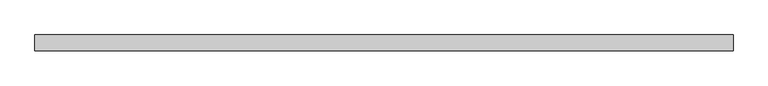
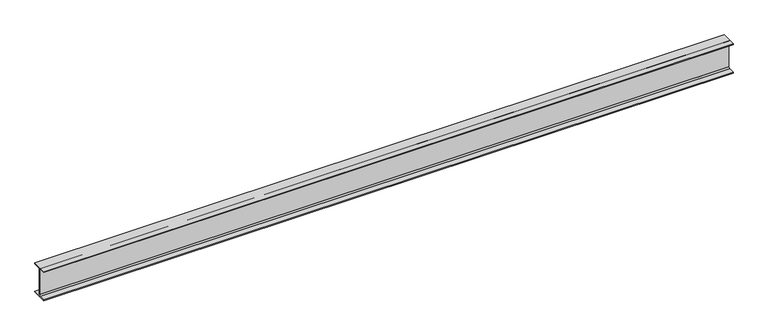
"""IFC4 building model written with IfcOpenShell, lengths in millimetres: beam geometry, Steel Framing_H_KS : H_SB_AR_S02_H-300x150x6.5x9_SRG3."""

import ifcopenshell
import ifcopenshell.guid

model = None  # the IFC model being written
_history = None  # IfcOwnerHistory: only IFC2X3 demands one
_inside = {}  # id of a spatial element -> (the spatial element, [elements in it])
_under = {}  # id of a project, library or spatial element -> (it, [spatial elements below it])
_declared = {}  # id of a project -> (the project, [libraries it declares])
_typed = {}  # id of a type object -> (the type object, [elements of that type])
_made_of = {}  # id of a material, layer set ... -> (it, [elements and type objects made of it])


def new_model(schema):
    """Start an empty IFC model of exactly this schema.

    Asked for "IFC4X3", IfcOpenShell would pick the latest addendum, in which some entities
    have other attributes; the version numbers below select the first issue.
    IFC2X3 requires an IfcOwnerHistory on every rooted entity: one is made here for all.
    """
    global model, _history
    if schema == "IFC4X3":
        model = ifcopenshell.file(schema_version=(4, 3, 0, 0))
    else:
        model = ifcopenshell.file(schema=schema)
    _inside.clear()
    _under.clear()
    _declared.clear()
    _typed.clear()
    _made_of.clear()
    _history = None
    if model.schema == "IFC2X3":
        org = make("IfcOrganization", Name="unknown")
        user = make(
            "IfcPersonAndOrganization",
            ThePerson=make("IfcPerson", FamilyName="unknown"),
            TheOrganization=org,
        )
        app = make(
            "IfcApplication",
            ApplicationDeveloper=org,
            Version="unknown",
            ApplicationFullName="unknown",
            ApplicationIdentifier="unknown",
        )
        _history = make(
            "IfcOwnerHistory",
            OwningUser=user,
            OwningApplication=app,
            ChangeAction="ADDED",
            CreationDate=0,
        )
    return model


def make(cls, **values):
    """One entity of the class cls with the attributes given. An attribute that is None is left unset."""
    return model.create_entity(
        cls, **{name: value for name, value in values.items() if value is not None}
    )


def rooted(cls, **values):
    """An entity with a GlobalId (a new one), such as an element, a storey or a relation."""
    return make(cls, GlobalId=ifcopenshell.guid.new(), OwnerHistory=_history, **values)


def si_unit(unit_type, name, prefix=None):
    """IfcSIUnit, for example si_unit("LENGTHUNIT", "METRE", prefix="MILLI")."""
    return make("IfcSIUnit", UnitType=unit_type, Prefix=prefix, Name=name)


def assignment(units):
    """IfcUnitAssignment: the units of a project."""
    return None if units is None else make("IfcUnitAssignment", Units=units)


def point(xyz):
    """IfcCartesianPoint."""
    return None if xyz is None else make("IfcCartesianPoint", Coordinates=xyz)


def direction(xyz):
    """IfcDirection."""
    return None if xyz is None else make("IfcDirection", DirectionRatios=xyz)


def frame(location, z_axis=None, x_axis=None):
    """IfcAxis2Placement3D, a coordinate frame: its origin and axes. An axis left out is left unset."""
    return make(
        "IfcAxis2Placement3D",
        Location=point(location),
        Axis=direction(z_axis),
        RefDirection=direction(x_axis),
    )


def frame_2d(location, x_axis=None):
    """IfcAxis2Placement2D, a coordinate frame in the plane: its origin and x axis."""
    return make(
        "IfcAxis2Placement2D", Location=point(location), RefDirection=direction(x_axis)
    )


def origin():
    """The frame at (0, 0, 0) with its axes left unset."""
    return frame((0.0, 0.0, 0.0))


def place(relative_to, where):
    """IfcLocalPlacement: puts the frame where relative to a parent placement (None: the world)."""
    return make(
        "IfcLocalPlacement", PlacementRelTo=relative_to, RelativePlacement=where
    )


def context(
    kind, dimensions, precision=None, world=None, true_north=None, identifier=None
):
    """IfcGeometricRepresentationContext, for example the 3D "Model" context."""
    return make(
        "IfcGeometricRepresentationContext",
        ContextIdentifier=identifier,
        ContextType=kind,
        CoordinateSpaceDimension=dimensions,
        Precision=precision,
        WorldCoordinateSystem=world,
        TrueNorth=true_north,
    )


def project(units=None, contexts=None):
    """IfcProject with its units and contexts."""
    return rooted(
        "IfcProject",
        Name="project",
        RepresentationContexts=contexts,
        UnitsInContext=assignment(units),
    )


def spatial(cls, under=None, at=None, **own):
    """A site, building, storey or space (cls), placed at a placement, below another one or the project."""
    s = rooted(cls, ObjectPlacement=at, **own)
    if under is not None:
        _under.setdefault(under.id(), (under, []))[1].append(s)
    return s


def polyline(points):
    """IfcPolyline through the points."""
    return make("IfcPolyline", Points=[point(p) for p in points])


def circle_curve(where, radius):
    """IfcCircle in the frame where."""
    return make("IfcCircle", Position=where, Radius=radius)


def trimmed(basis, trim1, trim2, sense, master):
    """IfcTrimmedCurve: the piece of a basis curve between two trims."""
    return make(
        "IfcTrimmedCurve",
        BasisCurve=basis,
        Trim1=trim1,
        Trim2=trim2,
        SenseAgreement=sense,
        MasterRepresentation=master,
    )


def segment(curve, same_sense, transition):
    """IfcCompositeCurveSegment."""
    return make(
        "IfcCompositeCurveSegment",
        Transition=transition,
        SameSense=same_sense,
        ParentCurve=curve,
    )


def composite_curve(segments, self_intersect=None):
    """IfcCompositeCurve: segments joined end to end."""
    return make("IfcCompositeCurve", Segments=segments, SelfIntersect=self_intersect)


def outline(outer, holes=None, kind="AREA"):
    """IfcArbitraryClosedProfileDef: a profile drawn as a closed curve; with holes, ...WithVoids."""
    if holes is None:
        return make("IfcArbitraryClosedProfileDef", ProfileType=kind, OuterCurve=outer)
    return make(
        "IfcArbitraryProfileDefWithVoids",
        ProfileType=kind,
        OuterCurve=outer,
        InnerCurves=holes,
    )


def extrude(swept, where, along, depth):
    """IfcExtrudedAreaSolid: the profile swept, set in the frame where, extruded along a direction by depth."""
    return make(
        "IfcExtrudedAreaSolid",
        SweptArea=swept,
        Position=where,
        ExtrudedDirection=direction(along),
        Depth=depth,
    )


def shape(context_of_items, identifier, shape_type, items):
    """IfcShapeRepresentation: the items that make up one representation, for example the "Body"."""
    return make(
        "IfcShapeRepresentation",
        ContextOfItems=context_of_items,
        RepresentationIdentifier=identifier,
        RepresentationType=shape_type,
        Items=items,
    )


def source(mapping_origin, context_of_items, identifier, shape_type, items):
    """IfcRepresentationMap: a shape defined once, which mapped items show again and again."""
    return make(
        "IfcRepresentationMap",
        MappingOrigin=mapping_origin,
        MappedRepresentation=shape(context_of_items, identifier, shape_type, items),
    )


def transform(
    local_origin,
    x_axis=None,
    y_axis=None,
    z_axis=None,
    scale=None,
    scale2=None,
    scale3=None,
    uniform=True,
):
    """IfcCartesianTransformationOperator3D, or its non-uniform kind. x_axis, y_axis, z_axis: its Axis1, 2, 3."""
    if uniform:
        return make(
            "IfcCartesianTransformationOperator3D",
            Axis1=direction(x_axis),
            Axis2=direction(y_axis),
            LocalOrigin=point(local_origin),
            Scale=scale,
            Axis3=direction(z_axis),
        )
    return make(
        "IfcCartesianTransformationOperator3DnonUniform",
        Axis1=direction(x_axis),
        Axis2=direction(y_axis),
        LocalOrigin=point(local_origin),
        Scale=scale,
        Axis3=direction(z_axis),
        Scale2=scale2,
        Scale3=scale3,
    )


def mapped(mapping_source, mapping_target):
    """IfcMappedItem: shows the shape of a source again, moved by a transform."""
    return make(
        "IfcMappedItem", MappingSource=mapping_source, MappingTarget=mapping_target
    )


def made_of(thing, what):
    """Note that an element or type object is made of a material, layer set ...; save() writes the relation."""
    if what is not None:
        _made_of.setdefault(what.id(), (what, []))[1].append(thing)
    return thing


def element(
    cls,
    number,
    at=None,
    inside=None,
    cuts=None,
    type_object=None,
    material=None,
    context=None,
    identifier="Body",
    shape_type=None,
    held_by="IfcProductDefinitionShape",
    body=None,
    shapes=None,
    **own,
):
    """One element of the class cls, such as IfcWall. Its Tag is "e" and its number.

    at: its placement. inside: the storey or other place that contains it. cuts: it is an
    opening in that element (IfcRelVoidsElement). A single representation is given by context,
    identifier, shape_type and body (its items); several are given by shapes. held_by: the class
    of the entity that holds the representations. save() writes the other relations.
    """
    e = rooted(cls, Tag="e%d" % number, ObjectPlacement=at, **own)
    if body is not None:
        shapes = [shape(context, identifier, shape_type, body)]
    if shapes is not None:
        e.Representation = make(held_by, Representations=shapes)
    if inside is not None:
        _inside.setdefault(inside.id(), (inside, []))[1].append(e)
    if cuts is not None:
        rooted(
            "IfcRelVoidsElement", RelatingBuildingElement=cuts, RelatedOpeningElement=e
        )
    if type_object is not None:
        _typed.setdefault(type_object.id(), (type_object, []))[1].append(e)
    return made_of(e, material)


def aggregate(whole, parts):
    """IfcRelAggregates: a whole, such as a stair, and the parts it consists of."""
    return rooted("IfcRelAggregates", RelatingObject=whole, RelatedObjects=parts)


def save(model, path):
    """Write the relations noted so far, then the file.

    IfcRelAggregates (storeys below a building ...), IfcRelContainedInSpatialStructure (elements
    in a storey), IfcRelDefinesByType, IfcRelAssociatesMaterial and IfcRelDeclares: one each for
    every whole, place, type object, material and project.
    """
    for whole, parts in _under.values():
        aggregate(whole, parts)
    for where, things in _inside.values():
        rooted(
            "IfcRelContainedInSpatialStructure",
            RelatedElements=things,
            RelatingStructure=where,
        )
    for kind, things in _typed.values():
        rooted("IfcRelDefinesByType", RelatedObjects=things, RelatingType=kind)
    for what, things in _made_of.values():
        rooted("IfcRelAssociatesMaterial", RelatedObjects=things, RelatingMaterial=what)
    for by, libraries in _declared.values():
        rooted("IfcRelDeclares", RelatingContext=by, RelatedDefinitions=libraries)
    model.write(path)


def beam_185c3a5d(model_context):
    return source(origin(), model_context, "Body", "SweptSolid", [
        extrude(outline(composite_curve([segment(polyline([(75.0, -141.0), (75.0, -150.0), (-75.0, -150.0), (-75.0, -141.0), (-16.25, -141.0)]), True, "CONTINUOUS"), segment(trimmed(circle_curve(frame_2d((-16.25, -128.0)), 13.0), [point((-16.25, -141.0))], [point((-3.25, -128.0))], True, "CARTESIAN"), True, "CONTINUOUS"), segment(polyline([(-3.25, -128.0), (-3.25, 128.0)]), True, "CONTINUOUS"), segment(trimmed(circle_curve(frame_2d((-16.25, 128.0)), 13.0), [point((-3.25, 128.0))], [point((-16.25, 141.0))], True, "CARTESIAN"), True, "CONTINUOUS"), segment(polyline([(-16.25, 141.0), (-75.0, 141.0), (-75.0, 150.0), (75.0, 150.0), (75.0, 141.0), (16.25, 141.0)]), True, "CONTINUOUS"), segment(trimmed(circle_curve(frame_2d((16.25, 128.0)), 13.0), [point((16.25, 141.0))], [point((3.25, 128.0))], True, "CARTESIAN"), True, "CONTINUOUS"), segment(polyline([(3.25, 128.0), (3.25, -128.0)]), True, "CONTINUOUS"), segment(trimmed(circle_curve(frame_2d((16.25, -128.0)), 13.0), [point((3.25, -128.0))], [point((16.25, -141.0))], True, "CARTESIAN"), True, "CONTINUOUS"), segment(polyline([(16.25, -141.0), (75.0, -141.0)]), True, "CONTINUOUS")], self_intersect=False)), frame((-3337.3, 0.0, 0.0), z_axis=(1.0, 0.0, 0.0), x_axis=(0.0, 1.0, 0.0)), (0.0, 0.0, 1.0), 6674.6),
    ])


if __name__ == "__main__":
    model = new_model("IFC4")
    model_context = context("Model", 3, world=origin())
    ifc_project = project(units=[si_unit("LENGTHUNIT", "METRE", prefix="MILLI")], contexts=[model_context])
    site = spatial("IfcSite", under=ifc_project)
    building = spatial("IfcBuilding", under=site)
    placement = place(None, origin())
    beam_shape = beam_185c3a5d(model_context)
    element("IfcBeam", 1, ObjectType="Steel Framing_H_KS : H_SB_AR_S02_H-300x150x6.5x9_SRG3", at=placement, inside=building, context=model_context, shape_type="MappedRepresentation", body=[
        mapped(beam_shape, transform((0.0, 0.0, 0.0), x_axis=(1.0, 0.0, 0.0), y_axis=(0.0, 1.0, 0.0), z_axis=(0.0, 0.0, 1.0))),
    ])
    save(model, "model.ifc")

# Revit data of these elements
# Type "Steel Framing_H_KS : H_SB_AR_S02_H-300x150x6.5x9_SRG3"
#   Type Comments = "MAIN"
#   Type Mark = "SRG3"
#   H_SectionID = "H-300x150x6.5x9"
#   H_Ratio for Additional Steel Plate = 0.2
#   Width = 15.0 cm
#   Web Thickness = 0.65 cm
#   Web Fillet = 1.3 cm
#   Warping Constant = 107000.0 cm⁶
#   Torsional Moment of Inertia = 9.9539 cm⁴
#   Section Area = 46.78 cm²
#   Plastic Modulus weak axis = 105.0 cm³
#   Plastic Modulus strong axis = 542.0 cm³
#   Perimeter = 1.17 m²/m
#   Nominal Weight = 36.70 kgf/m
#   Moment of Inertia weak axis = 508.00 cm⁴
#   Moment of Inertia strong axis = 7210.00 cm⁴
#   Height = 30.0 cm
#   Flange Thickness = 0.9 cm
#   Elastic Modulus weak axis = 67.7 cm³
#   Elastic Modulus strong axis = 481.0 cm³
#   Centroid Vertical = 15.0 cm
#   Centroid Horizontal = 7.5 cm
#   Bolt Spacing = 8.89 cm
#   Length [instance default] = 1500 mm
#   Structural Material [instance default] = Steel, 45-345
#   Section Name Key = ""
#   Assembly Code = ""
# Element 1 (IfcBeam, "Steel Framing_H_KS : H_SB_AR_S02_H-300x150x6.5x9_SRG3")
#   Materials on its faces: "Steel, 45-345"
# Materials
#   "Steel, 45-345": class "Metal", colour RGB 189 187 185, transparency 0, Description = "Steel 345 MPa", Cost = 0
